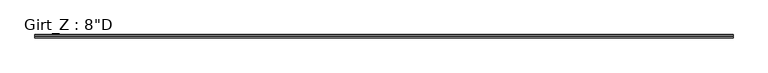
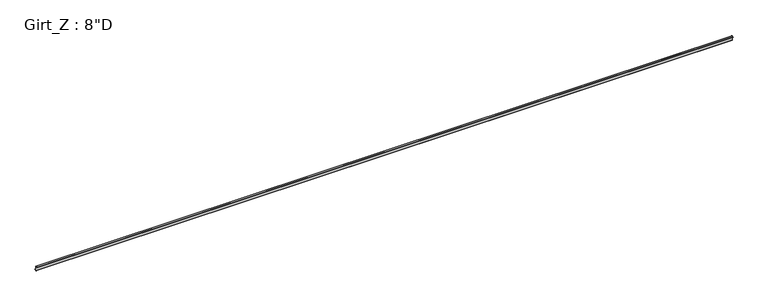
"""IFC4 building model written with IfcOpenShell, lengths in millimetres: beam geometry."""

from ifc_helpers import new_model, si_unit, point, frame, frame_2d, origin, place, context, project, spatial, polyline, circle_curve, trimmed, segment, composite_curve, outline, extrude, source, transform, mapped, element, save


def beam_797c0845(model_context):
    return source(origin(), model_context, "Body", "SweptSolid", [
        extrude(outline(composite_curve([segment(polyline([(-63.5, 101.6), (-3.3734375, 101.6)]), True, "CONTINUOUS"), segment(trimmed(circle_curve(frame_2d((-3.3734375, 96.8375)), 4.7625), [point((-3.3734375, 101.6))], [point((1.3890625, 96.8375))], False, "CARTESIAN"), True, "CONTINUOUS"), segment(polyline([(1.3890625, 96.8375), (1.3890625, -96.8389339)]), True, "CONTINUOUS"), segment(trimmed(circle_curve(frame_2d((3.3748024, -96.8389339)), 1.9857399), [point((1.3890625, -96.8389339))], [point((3.2694106, -98.821875))], True, "CARTESIAN"), True, "CONTINUOUS"), segment(polyline([(3.2694106, -98.821875), (62.204539, -98.821875), (73.6169367, -85.221109), (75.745104, -87.0068534), (63.5, -101.6), (3.3734375, -101.6)]), True, "CONTINUOUS"), segment(trimmed(circle_curve(frame_2d((3.3734375, -96.8375)), 4.7625), [point((3.3734375, -101.6))], [point((-1.3890625, -96.8375))], False, "CARTESIAN"), True, "CONTINUOUS"), segment(polyline([(-1.3890625, -96.8375), (-1.3890625, 96.8381931)]), True, "CONTINUOUS"), segment(trimmed(circle_curve(frame_2d((-3.3741066, 96.8381931)), 1.9850441), [point((-1.3890625, 96.8381931))], [point((-3.3005807, 98.821875))], True, "CARTESIAN"), True, "CONTINUOUS"), segment(polyline([(-3.3005807, 98.821875), (-62.204539, 98.821875), (-73.6169367, 85.221109), (-75.745104, 87.0068534), (-63.5, 101.6)]), True, "CONTINUOUS")], self_intersect=False)), frame((-15693.23125, 0.0, 0.0), z_axis=(1.0, 0.0, 0.0), x_axis=(0.0, 1.0, 0.0)), (0.0, 0.0, 1.0), 31219.775),
    ])


if __name__ == "__main__":
    model = new_model("IFC4")
    model_context = context("Model", 3, world=origin())
    ifc_project = project(units=[si_unit("LENGTHUNIT", "METRE", prefix="MILLI")], contexts=[model_context])
    site = spatial("IfcSite", under=ifc_project)
    building = spatial("IfcBuilding", under=site)
    placement = place(None, origin())
    beam_shape = beam_797c0845(model_context)
    element("IfcBeam", 1, ObjectType="Girt_Z : 8\"D", at=placement, inside=building, context=model_context, shape_type="MappedRepresentation", body=[
        mapped(beam_shape, transform((0.0, 0.0, 0.0), x_axis=(1.0, 0.0, 0.0), y_axis=(0.0, 1.0, 0.0), z_axis=(0.0, 0.0, 1.0))),
    ])
    save(model, "model.ifc")

# Revit data of these elements
# Type "Girt_Z : 8\"D"
#   Web_Thickness = 0' - 0 7/64"
#   Length [instance default] = 10' - 0"
#   Leg_1 = 0' - 2 1/2"
#   Height = 0' - 8"
#   Structural Material [instance default] = none
# Element 1 (IfcBeam, "Girt_Z : 8\"D")
#   Structural Material = Steel
#   Materials on its faces: "Steel"
# Materials
#   "Steel": class "Metal", colour RGB 118 118 114, transparency 0, Description = "Steel, mill finish", Cost = 0
